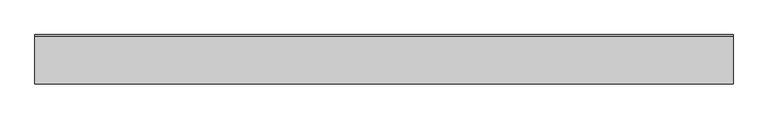
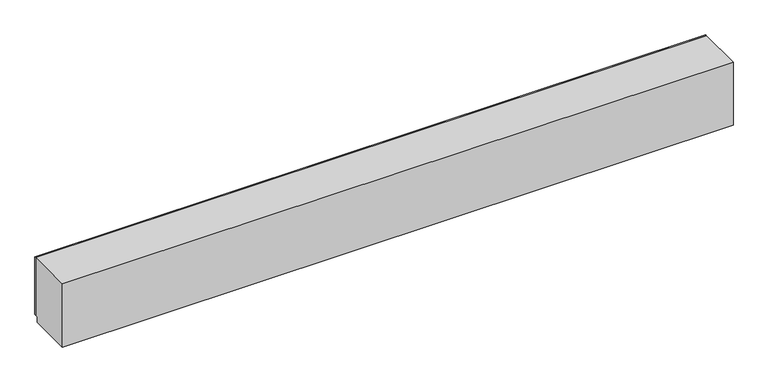
"""IFC4 building model written with IfcOpenShell, lengths in millimetres: furniture geometry, OD_CW_Base Cabinet : OD_CW_Base Cabinet."""

from ifc_helpers import new_model, si_unit, frame, origin, place, context, project, spatial, polyline, outline, extrude, source, transform, mapped, element, save


def furniture_c99718ca(model_context):
    return source(origin(), model_context, "Body", "SweptSolid", [
        extrude(outline(polyline([(18.7377049, 228.6), (18.7377049, 254.0), (12195.519328, 254.0), (12195.519328, 228.6), (18.7377049, 228.6)])), frame((0.0, 0.0, 101.6), z_axis=(0.0, 0.0, 1.0), x_axis=(1.0, 0.0, 0.0)), (0.0, 0.0, 1.0), 1112.7587451),
        extrude(outline(polyline([(228.6, 1214.3587451), (228.6, 101.6), (177.8, 101.6), (177.8, 0.0), (-609.6, 0.0), (-609.6, 1214.3587451), (228.6, 1214.3587451)])), frame((18.7377049, 0.0, 0.0), z_axis=(1.0, 0.0, 0.0), x_axis=(0.0, 1.0, 0.0)), (0.0, 0.0, 1.0), 12176.7816231),
    ])


if __name__ == "__main__":
    model = new_model("IFC4")
    model_context = context("Model", 3, world=origin())
    ifc_project = project(units=[si_unit("LENGTHUNIT", "METRE", prefix="MILLI")], contexts=[model_context])
    site = spatial("IfcSite", under=ifc_project)
    building = spatial("IfcBuilding", under=site)
    placement = place(None, origin())
    furniture_shape = furniture_c99718ca(model_context)
    element("IfcFurniture", 1, ObjectType="OD_CW_Base Cabinet : OD_CW_Base Cabinet", at=placement, inside=building, context=model_context, shape_type="MappedRepresentation", body=[
        mapped(furniture_shape, transform((0.0, 0.0, 0.0), x_axis=(1.0, 0.0, 0.0), y_axis=(0.0, 1.0, 0.0), z_axis=(0.0, 0.0, 1.0))),
    ])
    save(model, "model.ifc")

# Revit data of these elements
# Type "OD_CW_Base Cabinet : OD_CW_Base Cabinet"
#   OD_CW_Width [instance default] = 2' - 10"
#   OD_CW_Length [instance default] = 8' - 0"
#   OD_CW_Height [instance default] = 2' - 3"
#   Depth = 2' - 0"
#   Height = 3' - 0"
#   Width = 4' - 0"
#   OD_CW_Material_Front Panel [instance default] = none
#   OD_CW_Material_Body [instance default] = none
# Element 1 (IfcFurniture, "OD_CW_Base Cabinet : OD_CW_Base Cabinet")
#   OD_CW_Length = 39' - 11.40085"
#   OD_CW_Height = 3' - 11.8094"
#   OD_CW_Material_Front Panel = WOOD-OAKFIRE
#   OD_CW_Material_Body = WOOD-OAKFIRE
#   Materials on its faces: "WOOD-OAKFIRE"
# Materials
#   "WOOD-OAKFIRE": class "Wood", colour RGB 198 202 183, transparency 0, Description = "Generic wood", Cost = 0
